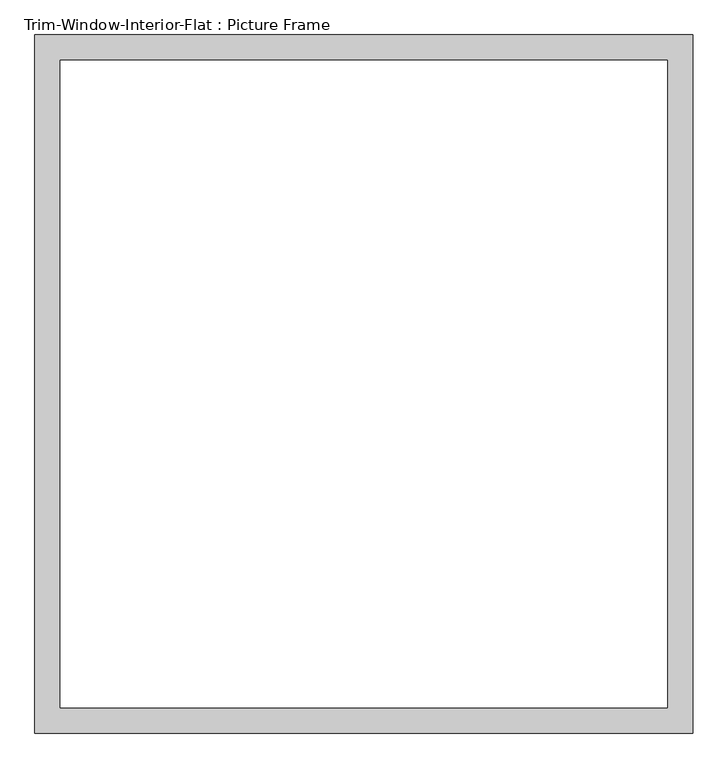
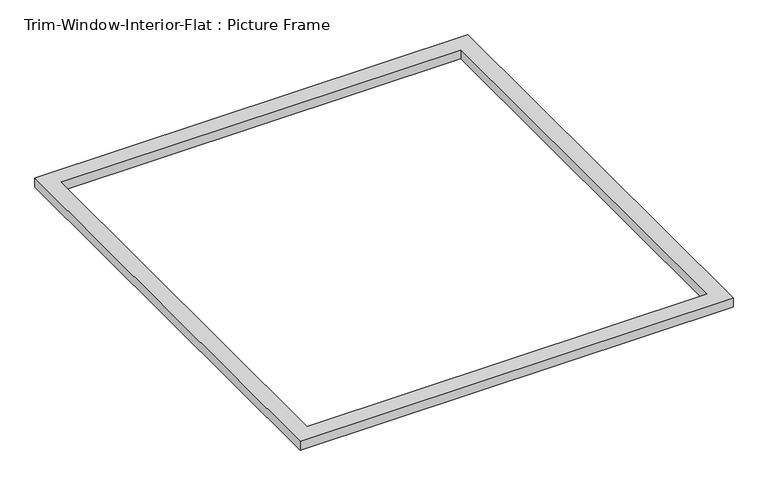
"""IFC4 building model written with IfcOpenShell, lengths in millimetres: proxy geometry, Trim-Window-Interior-Flat : Picture Frame."""

from ifc_helpers import new_model, si_unit, origin, origin_with_axes, place, context, project, spatial, polyline, outline, extrude, source, transform, mapped, element, save


def trim_window_interior_flat_picture_frame_f9059606(model_context):
    return source(origin(), model_context, "Body", "SweptSolid", [
        extrude(outline(polyline([(736.6, 44.45), (736.6, -1517.65), (-736.6, -1517.65), (-736.6, 44.45), (736.6, 44.45)]), holes=[polyline([(679.45, -12.7), (-679.45, -12.7), (-679.45, -1460.5), (679.45, -1460.5), (679.45, -12.7)])]), origin_with_axes(), (0.0, 0.0, 1.0), 31.75),
    ])


if __name__ == "__main__":
    model = new_model("IFC4")
    model_context = context("Model", 3, world=origin())
    ifc_project = project(units=[si_unit("LENGTHUNIT", "METRE", prefix="MILLI")], contexts=[model_context])
    site = spatial("IfcSite", under=ifc_project)
    building = spatial("IfcBuilding", under=site)
    placement = place(None, origin())
    trim_window_interior_flat_picture_frame_shape = trim_window_interior_flat_picture_frame_f9059606(model_context)
    element("IfcBuildingElementProxy", 1, Name="Trim-Window-Interior-Flat : Picture Frame", ObjectType="Trim-Window-Interior-Flat : Picture Frame", at=placement, inside=building, context=model_context, shape_type="MappedRepresentation", body=[
        mapped(trim_window_interior_flat_picture_frame_shape, transform((0.0, 0.0, 0.0), x_axis=(1.0, 0.0, 0.0), y_axis=(0.0, 1.0, 0.0), z_axis=(0.0, 0.0, 1.0))),
    ])
    save(model, "model.ifc")

# Revit data of these elements
# Type "Trim-Window-Interior-Flat : Picture Frame"
#   Trim Thickness_Picture Frame = 0' - 1 1/4"
#   Trim Width = 0' - 2 1/4"
#   Trim Thickness_with Sill = 0' - 0 3/4"
#   Sill Thickness = 0' - 1 1/4"
#   Opening Width [instance default] = 2' - 0"
#   Opening Height [instance default] = 3' - 0"
#   Default Elevation = 4' - 0"
#   Sill = no
#   Picture Frame = yes
#   Trim Material [instance default] = none
# Element 1 (IfcBuildingElementProxy, "Trim-Window-Interior-Flat : Picture Frame")
#   Opening Width = 4' - 6 1/2"
#   Opening Height = 4' - 10"
#   Trim Material = 1X WOOD COMPOSITE TRIM
#   Materials on its faces: "1X WOOD COMPOSITE TRIM"
# Materials
#   "1X WOOD COMPOSITE TRIM": class "Generic", colour RGB 88 61 61, transparency 0, Cost = 0
